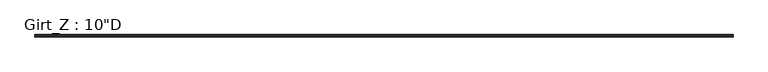
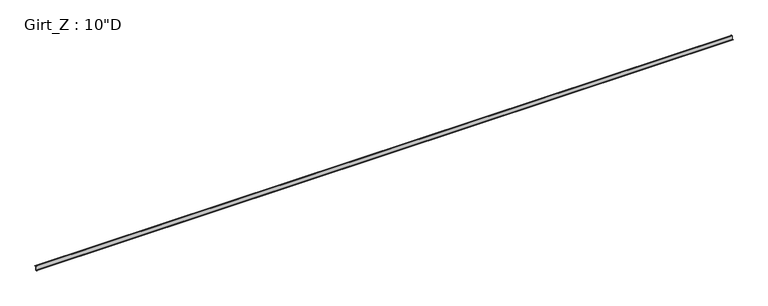
"""IFC4 building model written with IfcOpenShell, lengths in millimetres: beam geometry."""

from ifc_helpers import new_model, si_unit, point, frame, frame_2d, origin, place, context, project, spatial, polyline, circle_curve, trimmed, segment, composite_curve, outline, extrude, source, transform, mapped, element, save


def beam_884d35ae(model_context):
    return source(origin(), model_context, "Body", "SweptSolid", [
        extrude(outline(composite_curve([segment(polyline([(63.5, 127.0), (75.745104, 112.4068534), (73.6169367, 110.621109), (62.204539, 124.221875), (3.3005807, 124.221875)]), True, "CONTINUOUS"), segment(trimmed(circle_curve(frame_2d((3.3741066, 122.2381931)), 1.9850441), [point((3.3005807, 124.221875))], [point((1.3890625, 122.2381931))], True, "CARTESIAN"), True, "CONTINUOUS"), segment(polyline([(1.3890625, 122.2381931), (1.3890625, -122.2375)]), True, "CONTINUOUS"), segment(trimmed(circle_curve(frame_2d((-3.3734375, -122.2375)), 4.7625), [point((1.3890625, -122.2375))], [point((-3.3734375, -127.0))], False, "CARTESIAN"), True, "CONTINUOUS"), segment(polyline([(-3.3734375, -127.0), (-63.5, -127.0), (-75.745104, -112.4068534), (-73.6169367, -110.621109), (-62.204539, -124.221875), (-3.2694106, -124.221875)]), True, "CONTINUOUS"), segment(trimmed(circle_curve(frame_2d((-3.3748024, -122.2389339)), 1.9857399), [point((-3.2694106, -124.221875))], [point((-1.3890625, -122.2389339))], True, "CARTESIAN"), True, "CONTINUOUS"), segment(polyline([(-1.3890625, -122.2389339), (-1.3890625, 122.2375)]), True, "CONTINUOUS"), segment(trimmed(circle_curve(frame_2d((3.3734375, 122.2375)), 4.7625), [point((-1.3890625, 122.2375))], [point((3.3734375, 127.0))], False, "CARTESIAN"), True, "CONTINUOUS"), segment(polyline([(3.3734375, 127.0), (63.5, 127.0)]), True, "CONTINUOUS")], self_intersect=False)), frame((-22098.0, 0.0, 0.0), z_axis=(1.0, 0.0, 0.0), x_axis=(0.0, 1.0, 0.0)), (0.0, 0.0, 1.0), 44025.82),
    ])


if __name__ == "__main__":
    model = new_model("IFC4")
    model_context = context("Model", 3, world=origin())
    ifc_project = project(units=[si_unit("LENGTHUNIT", "METRE", prefix="MILLI")], contexts=[model_context])
    site = spatial("IfcSite", under=ifc_project)
    building = spatial("IfcBuilding", under=site)
    placement = place(None, origin())
    beam_shape = beam_884d35ae(model_context)
    element("IfcBeam", 1, ObjectType="Girt_Z : 10\"D", at=placement, inside=building, context=model_context, shape_type="MappedRepresentation", body=[
        mapped(beam_shape, transform((0.0, 0.0, 0.0), x_axis=(1.0, 0.0, 0.0), y_axis=(0.0, 1.0, 0.0), z_axis=(0.0, 0.0, 1.0))),
    ])
    save(model, "model.ifc")

# Revit data of these elements
# Type "Girt_Z : 10\"D"
#   Web_Thickness = 0' - 0 7/64"
#   Length [instance default] = 10' - 0"
#   Leg_1 = 0' - 2 1/2"
#   Height = 0' - 10"
